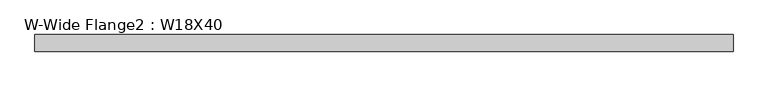
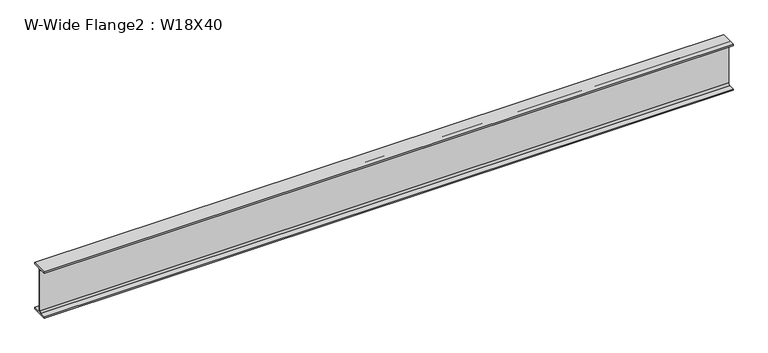
"""IFC4 building model written with IfcOpenShell, lengths in millimetres: beam geometry, W-Wide Flange2 : W18X40."""

import ifcopenshell
import ifcopenshell.guid

model = None  # the IFC model being written
_history = None  # IfcOwnerHistory: only IFC2X3 demands one
_inside = {}  # id of a spatial element -> (the spatial element, [elements in it])
_under = {}  # id of a project, library or spatial element -> (it, [spatial elements below it])
_declared = {}  # id of a project -> (the project, [libraries it declares])
_typed = {}  # id of a type object -> (the type object, [elements of that type])
_made_of = {}  # id of a material, layer set ... -> (it, [elements and type objects made of it])


def new_model(schema):
    """Start an empty IFC model of exactly this schema.

    Asked for "IFC4X3", IfcOpenShell would pick the latest addendum, in which some entities
    have other attributes; the version numbers below select the first issue.
    IFC2X3 requires an IfcOwnerHistory on every rooted entity: one is made here for all.
    """
    global model, _history
    if schema == "IFC4X3":
        model = ifcopenshell.file(schema_version=(4, 3, 0, 0))
    else:
        model = ifcopenshell.file(schema=schema)
    _inside.clear()
    _under.clear()
    _declared.clear()
    _typed.clear()
    _made_of.clear()
    _history = None
    if model.schema == "IFC2X3":
        org = make("IfcOrganization", Name="unknown")
        user = make(
            "IfcPersonAndOrganization",
            ThePerson=make("IfcPerson", FamilyName="unknown"),
            TheOrganization=org,
        )
        app = make(
            "IfcApplication",
            ApplicationDeveloper=org,
            Version="unknown",
            ApplicationFullName="unknown",
            ApplicationIdentifier="unknown",
        )
        _history = make(
            "IfcOwnerHistory",
            OwningUser=user,
            OwningApplication=app,
            ChangeAction="ADDED",
            CreationDate=0,
        )
    return model


def make(cls, **values):
    """One entity of the class cls with the attributes given. An attribute that is None is left unset."""
    return model.create_entity(
        cls, **{name: value for name, value in values.items() if value is not None}
    )


def rooted(cls, **values):
    """An entity with a GlobalId (a new one), such as an element, a storey or a relation."""
    return make(cls, GlobalId=ifcopenshell.guid.new(), OwnerHistory=_history, **values)


def si_unit(unit_type, name, prefix=None):
    """IfcSIUnit, for example si_unit("LENGTHUNIT", "METRE", prefix="MILLI")."""
    return make("IfcSIUnit", UnitType=unit_type, Prefix=prefix, Name=name)


def assignment(units):
    """IfcUnitAssignment: the units of a project."""
    return None if units is None else make("IfcUnitAssignment", Units=units)


def point(xyz):
    """IfcCartesianPoint."""
    return None if xyz is None else make("IfcCartesianPoint", Coordinates=xyz)


def direction(xyz):
    """IfcDirection."""
    return None if xyz is None else make("IfcDirection", DirectionRatios=xyz)


def frame(location, z_axis=None, x_axis=None):
    """IfcAxis2Placement3D, a coordinate frame: its origin and axes. An axis left out is left unset."""
    return make(
        "IfcAxis2Placement3D",
        Location=point(location),
        Axis=direction(z_axis),
        RefDirection=direction(x_axis),
    )


def frame_2d(location, x_axis=None):
    """IfcAxis2Placement2D, a coordinate frame in the plane: its origin and x axis."""
    return make(
        "IfcAxis2Placement2D", Location=point(location), RefDirection=direction(x_axis)
    )


def origin():
    """The frame at (0, 0, 0) with its axes left unset."""
    return frame((0.0, 0.0, 0.0))


def place(relative_to, where):
    """IfcLocalPlacement: puts the frame where relative to a parent placement (None: the world)."""
    return make(
        "IfcLocalPlacement", PlacementRelTo=relative_to, RelativePlacement=where
    )


def context(
    kind, dimensions, precision=None, world=None, true_north=None, identifier=None
):
    """IfcGeometricRepresentationContext, for example the 3D "Model" context."""
    return make(
        "IfcGeometricRepresentationContext",
        ContextIdentifier=identifier,
        ContextType=kind,
        CoordinateSpaceDimension=dimensions,
        Precision=precision,
        WorldCoordinateSystem=world,
        TrueNorth=true_north,
    )


def project(units=None, contexts=None):
    """IfcProject with its units and contexts."""
    return rooted(
        "IfcProject",
        Name="project",
        RepresentationContexts=contexts,
        UnitsInContext=assignment(units),
    )


def spatial(cls, under=None, at=None, **own):
    """A site, building, storey or space (cls), placed at a placement, below another one or the project."""
    s = rooted(cls, ObjectPlacement=at, **own)
    if under is not None:
        _under.setdefault(under.id(), (under, []))[1].append(s)
    return s


def polyline(points):
    """IfcPolyline through the points."""
    return make("IfcPolyline", Points=[point(p) for p in points])


def circle_curve(where, radius):
    """IfcCircle in the frame where."""
    return make("IfcCircle", Position=where, Radius=radius)


def trimmed(basis, trim1, trim2, sense, master):
    """IfcTrimmedCurve: the piece of a basis curve between two trims."""
    return make(
        "IfcTrimmedCurve",
        BasisCurve=basis,
        Trim1=trim1,
        Trim2=trim2,
        SenseAgreement=sense,
        MasterRepresentation=master,
    )


def segment(curve, same_sense, transition):
    """IfcCompositeCurveSegment."""
    return make(
        "IfcCompositeCurveSegment",
        Transition=transition,
        SameSense=same_sense,
        ParentCurve=curve,
    )


def composite_curve(segments, self_intersect=None):
    """IfcCompositeCurve: segments joined end to end."""
    return make("IfcCompositeCurve", Segments=segments, SelfIntersect=self_intersect)


def outline(outer, holes=None, kind="AREA"):
    """IfcArbitraryClosedProfileDef: a profile drawn as a closed curve; with holes, ...WithVoids."""
    if holes is None:
        return make("IfcArbitraryClosedProfileDef", ProfileType=kind, OuterCurve=outer)
    return make(
        "IfcArbitraryProfileDefWithVoids",
        ProfileType=kind,
        OuterCurve=outer,
        InnerCurves=holes,
    )


def extrude(swept, where, along, depth):
    """IfcExtrudedAreaSolid: the profile swept, set in the frame where, extruded along a direction by depth."""
    return make(
        "IfcExtrudedAreaSolid",
        SweptArea=swept,
        Position=where,
        ExtrudedDirection=direction(along),
        Depth=depth,
    )


def shape(context_of_items, identifier, shape_type, items):
    """IfcShapeRepresentation: the items that make up one representation, for example the "Body"."""
    return make(
        "IfcShapeRepresentation",
        ContextOfItems=context_of_items,
        RepresentationIdentifier=identifier,
        RepresentationType=shape_type,
        Items=items,
    )


def source(mapping_origin, context_of_items, identifier, shape_type, items):
    """IfcRepresentationMap: a shape defined once, which mapped items show again and again."""
    return make(
        "IfcRepresentationMap",
        MappingOrigin=mapping_origin,
        MappedRepresentation=shape(context_of_items, identifier, shape_type, items),
    )


def transform(
    local_origin,
    x_axis=None,
    y_axis=None,
    z_axis=None,
    scale=None,
    scale2=None,
    scale3=None,
    uniform=True,
):
    """IfcCartesianTransformationOperator3D, or its non-uniform kind. x_axis, y_axis, z_axis: its Axis1, 2, 3."""
    if uniform:
        return make(
            "IfcCartesianTransformationOperator3D",
            Axis1=direction(x_axis),
            Axis2=direction(y_axis),
            LocalOrigin=point(local_origin),
            Scale=scale,
            Axis3=direction(z_axis),
        )
    return make(
        "IfcCartesianTransformationOperator3DnonUniform",
        Axis1=direction(x_axis),
        Axis2=direction(y_axis),
        LocalOrigin=point(local_origin),
        Scale=scale,
        Axis3=direction(z_axis),
        Scale2=scale2,
        Scale3=scale3,
    )


def mapped(mapping_source, mapping_target):
    """IfcMappedItem: shows the shape of a source again, moved by a transform."""
    return make(
        "IfcMappedItem", MappingSource=mapping_source, MappingTarget=mapping_target
    )


def made_of(thing, what):
    """Note that an element or type object is made of a material, layer set ...; save() writes the relation."""
    if what is not None:
        _made_of.setdefault(what.id(), (what, []))[1].append(thing)
    return thing


def element(
    cls,
    number,
    at=None,
    inside=None,
    cuts=None,
    type_object=None,
    material=None,
    context=None,
    identifier="Body",
    shape_type=None,
    held_by="IfcProductDefinitionShape",
    body=None,
    shapes=None,
    **own,
):
    """One element of the class cls, such as IfcWall. Its Tag is "e" and its number.

    at: its placement. inside: the storey or other place that contains it. cuts: it is an
    opening in that element (IfcRelVoidsElement). A single representation is given by context,
    identifier, shape_type and body (its items); several are given by shapes. held_by: the class
    of the entity that holds the representations. save() writes the other relations.
    """
    e = rooted(cls, Tag="e%d" % number, ObjectPlacement=at, **own)
    if body is not None:
        shapes = [shape(context, identifier, shape_type, body)]
    if shapes is not None:
        e.Representation = make(held_by, Representations=shapes)
    if inside is not None:
        _inside.setdefault(inside.id(), (inside, []))[1].append(e)
    if cuts is not None:
        rooted(
            "IfcRelVoidsElement", RelatingBuildingElement=cuts, RelatedOpeningElement=e
        )
    if type_object is not None:
        _typed.setdefault(type_object.id(), (type_object, []))[1].append(e)
    return made_of(e, material)


def aggregate(whole, parts):
    """IfcRelAggregates: a whole, such as a stair, and the parts it consists of."""
    return rooted("IfcRelAggregates", RelatingObject=whole, RelatedObjects=parts)


def save(model, path):
    """Write the relations noted so far, then the file.

    IfcRelAggregates (storeys below a building ...), IfcRelContainedInSpatialStructure (elements
    in a storey), IfcRelDefinesByType, IfcRelAssociatesMaterial and IfcRelDeclares: one each for
    every whole, place, type object, material and project.
    """
    for whole, parts in _under.values():
        aggregate(whole, parts)
    for where, things in _inside.values():
        rooted(
            "IfcRelContainedInSpatialStructure",
            RelatedElements=things,
            RelatingStructure=where,
        )
    for kind, things in _typed.values():
        rooted("IfcRelDefinesByType", RelatedObjects=things, RelatingType=kind)
    for what, things in _made_of.values():
        rooted("IfcRelAssociatesMaterial", RelatedObjects=things, RelatingMaterial=what)
    for by, libraries in _declared.values():
        rooted("IfcRelDeclares", RelatingContext=by, RelatedDefinitions=libraries)
    model.write(path)


def w_wide_flange2_w18x40_1ff26780(model_context):
    return source(origin(), model_context, "Body", "SweptSolid", [
        extrude(outline(composite_curve([segment(polyline([(76.454, -213.995), (76.454, -227.33), (-76.454, -227.33), (-76.454, -213.995), (-20.828, -213.995)]), True, "CONTINUOUS"), segment(trimmed(circle_curve(frame_2d((-20.828, -197.1675)), 16.8275), [point((-20.828, -213.995))], [point((-4.0005, -197.1675))], True, "CARTESIAN"), True, "CONTINUOUS"), segment(polyline([(-4.0005, -197.1675), (-4.0005, 197.1675)]), True, "CONTINUOUS"), segment(trimmed(circle_curve(frame_2d((-20.828, 197.1675)), 16.8275), [point((-4.0005, 197.1675))], [point((-20.828, 213.995))], True, "CARTESIAN"), True, "CONTINUOUS"), segment(polyline([(-20.828, 213.995), (-76.454, 213.995), (-76.454, 227.33), (76.454, 227.33), (76.454, 213.995), (20.828, 213.995)]), True, "CONTINUOUS"), segment(trimmed(circle_curve(frame_2d((20.828, 197.1675)), 16.8275), [point((20.828, 213.995))], [point((4.0005, 197.1675))], True, "CARTESIAN"), True, "CONTINUOUS"), segment(polyline([(4.0005, 197.1675), (4.0005, -197.1675)]), True, "CONTINUOUS"), segment(trimmed(circle_curve(frame_2d((20.828, -197.1675)), 16.8275), [point((4.0005, -197.1675))], [point((20.828, -213.995))], True, "CARTESIAN"), True, "CONTINUOUS"), segment(polyline([(20.828, -213.995), (76.454, -213.995)]), True, "CONTINUOUS")], self_intersect=False)), frame((-3206.353125, 0.0, 0.0), z_axis=(1.0, 0.0, 0.0), x_axis=(0.0, 1.0, 0.0)), (0.0, 0.0, 1.0), 6417.865625),
    ])


if __name__ == "__main__":
    model = new_model("IFC4")
    model_context = context("Model", 3, world=origin())
    ifc_project = project(units=[si_unit("LENGTHUNIT", "METRE", prefix="MILLI")], contexts=[model_context])
    site = spatial("IfcSite", under=ifc_project)
    building = spatial("IfcBuilding", under=site)
    placement = place(None, origin())
    w_wide_flange2_w18x40_shape = w_wide_flange2_w18x40_1ff26780(model_context)
    element("IfcBeam", 1, ObjectType="W-Wide Flange2 : W18X40", at=placement, inside=building, context=model_context, shape_type="MappedRepresentation", body=[
        mapped(w_wide_flange2_w18x40_shape, transform((0.0, 0.0, 0.0), x_axis=(1.0, 0.0, 0.0), y_axis=(0.0, 1.0, 0.0), z_axis=(0.0, 0.0, 1.0))),
    ])
    save(model, "model.ifc")

# Revit data of these elements
# Type "W-Wide Flange2 : W18X40"
#   Assembly Code = "B10"
#   W = 40
#   Length [instance default] = 5' - 0"
#   bf = 0' - 6.02"
#   d = 1' - 5.9"
#   k = 0' - 1 3/16"
#   k2 = 0' - 0.6625"
#   tf = 0' - 0.525"
#   tw = 0' - 0.315"
#   A = 0.0819444 SF
#   Structural Material [instance default] = Steel ASTM A992
# Element 1 (IfcBeam, "W-Wide Flange2 : W18X40")
#   Materials on its faces: "Steel ASTM A992"
# Materials
#   "Steel ASTM A992": class "Metal", colour RGB 199 199 199, transparency 0, Description = "Structural steel 50ksi", Cost = 0
